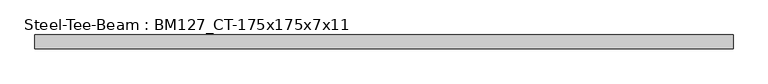
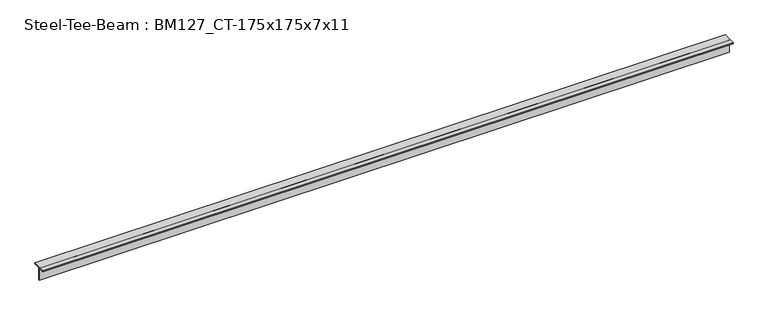
"""IFC4 building model written with IfcOpenShell, lengths in millimetres: beam geometry, Steel-Tee-Beam : BM127_CT-175x175x7x11."""

import ifcopenshell
import ifcopenshell.guid

model = None  # the IFC model being written
_history = None  # IfcOwnerHistory: only IFC2X3 demands one
_inside = {}  # id of a spatial element -> (the spatial element, [elements in it])
_under = {}  # id of a project, library or spatial element -> (it, [spatial elements below it])
_declared = {}  # id of a project -> (the project, [libraries it declares])
_typed = {}  # id of a type object -> (the type object, [elements of that type])
_made_of = {}  # id of a material, layer set ... -> (it, [elements and type objects made of it])


def new_model(schema):
    """Start an empty IFC model of exactly this schema.

    Asked for "IFC4X3", IfcOpenShell would pick the latest addendum, in which some entities
    have other attributes; the version numbers below select the first issue.
    IFC2X3 requires an IfcOwnerHistory on every rooted entity: one is made here for all.
    """
    global model, _history
    if schema == "IFC4X3":
        model = ifcopenshell.file(schema_version=(4, 3, 0, 0))
    else:
        model = ifcopenshell.file(schema=schema)
    _inside.clear()
    _under.clear()
    _declared.clear()
    _typed.clear()
    _made_of.clear()
    _history = None
    if model.schema == "IFC2X3":
        org = make("IfcOrganization", Name="unknown")
        user = make(
            "IfcPersonAndOrganization",
            ThePerson=make("IfcPerson", FamilyName="unknown"),
            TheOrganization=org,
        )
        app = make(
            "IfcApplication",
            ApplicationDeveloper=org,
            Version="unknown",
            ApplicationFullName="unknown",
            ApplicationIdentifier="unknown",
        )
        _history = make(
            "IfcOwnerHistory",
            OwningUser=user,
            OwningApplication=app,
            ChangeAction="ADDED",
            CreationDate=0,
        )
    return model


def make(cls, **values):
    """One entity of the class cls with the attributes given. An attribute that is None is left unset."""
    return model.create_entity(
        cls, **{name: value for name, value in values.items() if value is not None}
    )


def rooted(cls, **values):
    """An entity with a GlobalId (a new one), such as an element, a storey or a relation."""
    return make(cls, GlobalId=ifcopenshell.guid.new(), OwnerHistory=_history, **values)


def si_unit(unit_type, name, prefix=None):
    """IfcSIUnit, for example si_unit("LENGTHUNIT", "METRE", prefix="MILLI")."""
    return make("IfcSIUnit", UnitType=unit_type, Prefix=prefix, Name=name)


def assignment(units):
    """IfcUnitAssignment: the units of a project."""
    return None if units is None else make("IfcUnitAssignment", Units=units)


def point(xyz):
    """IfcCartesianPoint."""
    return None if xyz is None else make("IfcCartesianPoint", Coordinates=xyz)


def direction(xyz):
    """IfcDirection."""
    return None if xyz is None else make("IfcDirection", DirectionRatios=xyz)


def frame(location, z_axis=None, x_axis=None):
    """IfcAxis2Placement3D, a coordinate frame: its origin and axes. An axis left out is left unset."""
    return make(
        "IfcAxis2Placement3D",
        Location=point(location),
        Axis=direction(z_axis),
        RefDirection=direction(x_axis),
    )


def frame_2d(location, x_axis=None):
    """IfcAxis2Placement2D, a coordinate frame in the plane: its origin and x axis."""
    return make(
        "IfcAxis2Placement2D", Location=point(location), RefDirection=direction(x_axis)
    )


def origin():
    """The frame at (0, 0, 0) with its axes left unset."""
    return frame((0.0, 0.0, 0.0))


def place(relative_to, where):
    """IfcLocalPlacement: puts the frame where relative to a parent placement (None: the world)."""
    return make(
        "IfcLocalPlacement", PlacementRelTo=relative_to, RelativePlacement=where
    )


def context(
    kind, dimensions, precision=None, world=None, true_north=None, identifier=None
):
    """IfcGeometricRepresentationContext, for example the 3D "Model" context."""
    return make(
        "IfcGeometricRepresentationContext",
        ContextIdentifier=identifier,
        ContextType=kind,
        CoordinateSpaceDimension=dimensions,
        Precision=precision,
        WorldCoordinateSystem=world,
        TrueNorth=true_north,
    )


def project(units=None, contexts=None):
    """IfcProject with its units and contexts."""
    return rooted(
        "IfcProject",
        Name="project",
        RepresentationContexts=contexts,
        UnitsInContext=assignment(units),
    )


def spatial(cls, under=None, at=None, **own):
    """A site, building, storey or space (cls), placed at a placement, below another one or the project."""
    s = rooted(cls, ObjectPlacement=at, **own)
    if under is not None:
        _under.setdefault(under.id(), (under, []))[1].append(s)
    return s


def polyline(points):
    """IfcPolyline through the points."""
    return make("IfcPolyline", Points=[point(p) for p in points])


def circle_curve(where, radius):
    """IfcCircle in the frame where."""
    return make("IfcCircle", Position=where, Radius=radius)


def trimmed(basis, trim1, trim2, sense, master):
    """IfcTrimmedCurve: the piece of a basis curve between two trims."""
    return make(
        "IfcTrimmedCurve",
        BasisCurve=basis,
        Trim1=trim1,
        Trim2=trim2,
        SenseAgreement=sense,
        MasterRepresentation=master,
    )


def segment(curve, same_sense, transition):
    """IfcCompositeCurveSegment."""
    return make(
        "IfcCompositeCurveSegment",
        Transition=transition,
        SameSense=same_sense,
        ParentCurve=curve,
    )


def composite_curve(segments, self_intersect=None):
    """IfcCompositeCurve: segments joined end to end."""
    return make("IfcCompositeCurve", Segments=segments, SelfIntersect=self_intersect)


def outline(outer, holes=None, kind="AREA"):
    """IfcArbitraryClosedProfileDef: a profile drawn as a closed curve; with holes, ...WithVoids."""
    if holes is None:
        return make("IfcArbitraryClosedProfileDef", ProfileType=kind, OuterCurve=outer)
    return make(
        "IfcArbitraryProfileDefWithVoids",
        ProfileType=kind,
        OuterCurve=outer,
        InnerCurves=holes,
    )


def extrude(swept, where, along, depth):
    """IfcExtrudedAreaSolid: the profile swept, set in the frame where, extruded along a direction by depth."""
    return make(
        "IfcExtrudedAreaSolid",
        SweptArea=swept,
        Position=where,
        ExtrudedDirection=direction(along),
        Depth=depth,
    )


def shape(context_of_items, identifier, shape_type, items):
    """IfcShapeRepresentation: the items that make up one representation, for example the "Body"."""
    return make(
        "IfcShapeRepresentation",
        ContextOfItems=context_of_items,
        RepresentationIdentifier=identifier,
        RepresentationType=shape_type,
        Items=items,
    )


def source(mapping_origin, context_of_items, identifier, shape_type, items):
    """IfcRepresentationMap: a shape defined once, which mapped items show again and again."""
    return make(
        "IfcRepresentationMap",
        MappingOrigin=mapping_origin,
        MappedRepresentation=shape(context_of_items, identifier, shape_type, items),
    )


def transform(
    local_origin,
    x_axis=None,
    y_axis=None,
    z_axis=None,
    scale=None,
    scale2=None,
    scale3=None,
    uniform=True,
):
    """IfcCartesianTransformationOperator3D, or its non-uniform kind. x_axis, y_axis, z_axis: its Axis1, 2, 3."""
    if uniform:
        return make(
            "IfcCartesianTransformationOperator3D",
            Axis1=direction(x_axis),
            Axis2=direction(y_axis),
            LocalOrigin=point(local_origin),
            Scale=scale,
            Axis3=direction(z_axis),
        )
    return make(
        "IfcCartesianTransformationOperator3DnonUniform",
        Axis1=direction(x_axis),
        Axis2=direction(y_axis),
        LocalOrigin=point(local_origin),
        Scale=scale,
        Axis3=direction(z_axis),
        Scale2=scale2,
        Scale3=scale3,
    )


def mapped(mapping_source, mapping_target):
    """IfcMappedItem: shows the shape of a source again, moved by a transform."""
    return make(
        "IfcMappedItem", MappingSource=mapping_source, MappingTarget=mapping_target
    )


def made_of(thing, what):
    """Note that an element or type object is made of a material, layer set ...; save() writes the relation."""
    if what is not None:
        _made_of.setdefault(what.id(), (what, []))[1].append(thing)
    return thing


def element(
    cls,
    number,
    at=None,
    inside=None,
    cuts=None,
    type_object=None,
    material=None,
    context=None,
    identifier="Body",
    shape_type=None,
    held_by="IfcProductDefinitionShape",
    body=None,
    shapes=None,
    **own,
):
    """One element of the class cls, such as IfcWall. Its Tag is "e" and its number.

    at: its placement. inside: the storey or other place that contains it. cuts: it is an
    opening in that element (IfcRelVoidsElement). A single representation is given by context,
    identifier, shape_type and body (its items); several are given by shapes. held_by: the class
    of the entity that holds the representations. save() writes the other relations.
    """
    e = rooted(cls, Tag="e%d" % number, ObjectPlacement=at, **own)
    if body is not None:
        shapes = [shape(context, identifier, shape_type, body)]
    if shapes is not None:
        e.Representation = make(held_by, Representations=shapes)
    if inside is not None:
        _inside.setdefault(inside.id(), (inside, []))[1].append(e)
    if cuts is not None:
        rooted(
            "IfcRelVoidsElement", RelatingBuildingElement=cuts, RelatedOpeningElement=e
        )
    if type_object is not None:
        _typed.setdefault(type_object.id(), (type_object, []))[1].append(e)
    return made_of(e, material)


def aggregate(whole, parts):
    """IfcRelAggregates: a whole, such as a stair, and the parts it consists of."""
    return rooted("IfcRelAggregates", RelatingObject=whole, RelatedObjects=parts)


def save(model, path):
    """Write the relations noted so far, then the file.

    IfcRelAggregates (storeys below a building ...), IfcRelContainedInSpatialStructure (elements
    in a storey), IfcRelDefinesByType, IfcRelAssociatesMaterial and IfcRelDeclares: one each for
    every whole, place, type object, material and project.
    """
    for whole, parts in _under.values():
        aggregate(whole, parts)
    for where, things in _inside.values():
        rooted(
            "IfcRelContainedInSpatialStructure",
            RelatedElements=things,
            RelatingStructure=where,
        )
    for kind, things in _typed.values():
        rooted("IfcRelDefinesByType", RelatedObjects=things, RelatingType=kind)
    for what, things in _made_of.values():
        rooted("IfcRelAssociatesMaterial", RelatedObjects=things, RelatingMaterial=what)
    for by, libraries in _declared.values():
        rooted("IfcRelDeclares", RelatingContext=by, RelatedDefinitions=libraries)
    model.write(path)


def steel_tee_beam_bm127_ct_175x175x7x11_fc6d57d6(model_context):
    return source(origin(), model_context, "Body", "SweptSolid", [
        extrude(outline(composite_curve([segment(polyline([(-87.5, 87.5), (87.5, 87.5), (87.5, 76.5), (17.5, 76.5)]), True, "CONTINUOUS"), segment(trimmed(circle_curve(frame_2d((17.5, 62.5)), 14.0), [point((17.5, 76.5))], [point((3.5, 62.5))], True, "CARTESIAN"), True, "CONTINUOUS"), segment(polyline([(3.5, 62.5), (3.5, -87.5), (-3.5, -87.5), (-3.5, 62.5)]), True, "CONTINUOUS"), segment(trimmed(circle_curve(frame_2d((-17.5, 62.5)), 14.0), [point((-3.5, 62.5))], [point((-17.5, 76.5))], True, "CARTESIAN"), True, "CONTINUOUS"), segment(polyline([(-17.5, 76.5), (-87.5, 76.5), (-87.5, 87.5)]), True, "CONTINUOUS")], self_intersect=False)), frame((-4298.1792655, 0.0, 0.0), z_axis=(1.0, 0.0, 0.0), x_axis=(0.0, 1.0, 0.0)), (0.0, 0.0, 1.0), 8725.555017),
    ])


if __name__ == "__main__":
    model = new_model("IFC4")
    model_context = context("Model", 3, world=origin())
    ifc_project = project(units=[si_unit("LENGTHUNIT", "METRE", prefix="MILLI")], contexts=[model_context])
    site = spatial("IfcSite", under=ifc_project)
    building = spatial("IfcBuilding", under=site)
    placement = place(None, origin())
    steel_tee_beam_bm127_ct_175x175x7x11_shape = steel_tee_beam_bm127_ct_175x175x7x11_fc6d57d6(model_context)
    element("IfcBeam", 1, ObjectType="Steel-Tee-Beam : BM127_CT-175x175x7x11", at=placement, inside=building, context=model_context, shape_type="MappedRepresentation", body=[
        mapped(steel_tee_beam_bm127_ct_175x175x7x11_shape, transform((0.0, 0.0, 0.0), x_axis=(1.0, 0.0, 0.0), y_axis=(0.0, 1.0, 0.0), z_axis=(0.0, 0.0, 1.0))),
    ])
    save(model, "model.ifc")

# Revit data of these elements
# Type "Steel-Tee-Beam : BM127_CT-175x175x7x11"
#   Surface Area = 0.00 m²/m
#   Section Area = 31.57 cm²
#   Mass per Unit Length = 24.80 kg/m
#   Length [instance default] = 1524 mm
#   bf = 175 mm
#   d = 175 mm
#   k = 25 mm
#   kr = 14 mm
#   tf = 11 mm
#   tw = 7 mm
#   hec_material4 [instance default] = none
#   hec_material3 [instance default] = none
#   hec_material2 [instance default] = none
#   hec_material1 [instance default] = none
#   Structural Material [instance default] = Steel, 45-345
#   Assembly Code = ""
# Element 1 (IfcBeam, "Steel-Tee-Beam : BM127_CT-175x175x7x11")
#   hec_material3 = F01AC000-00002_Building/Shelter Fire Proofing Work_Intumescent Coating Type_1 hr. rating (UL 1709))
#   hec_material2 = S01AA010-00002_Main Steel Structure Fabrication Work_Shelter/Building_Steel Painting/Coating_for Fireproofed Steel Surface, Surface Preparation & Primer Coat
#   hec_material1 = S03AA029-00001_Main Steel Structure Erection Work_Shelter/Building_Light Steel
#   Structural Material = S01AA003-00001_Main Steel Structure Fabrication Work_Shelter/Building_Light Steel - Standard
#   Materials on its faces: "S01AA003-00001_Main Steel Structure Fabrication Work_Shelter/Building_Light Steel - Standard"
# Materials
#   "Steel, 45-345": class "Metal", colour RGB 189 187 185, transparency 0, Description = "Steel 345 MPa", Cost = 0
#   "S01AA003-00001_Main Steel Structure Fabrication Work_Shelter/Building_Light Steel - Standard": class "Metal", colour RGB 120 120 120, transparency 0, Comments = "(30KG/M>Weight)", Description = "Structural steel 50ksi", W00) Work Master Code = "S01AA003-00001", W01) Work Master_Lv1 = "Main Steel Structure Fabrication Work", W02) Work Master_Lv2 = "Shelter/Building", W03) Work Master_Spec.1 = "Light Steel - Standard (30KG/M>Weight)", Cost = 0
#   "F01AC000-00002_Building/Shelter Fire Proofing Work_Intumescent Coating Type_1 hr. rating (UL 1709))": class "Metal", colour RGB 255 128 128, transparency 0, Description = "Paint finished steel", W00) Work Master Code = "F01AC000-00002", W01) Work Master_Lv1 = "Building/Shelter Fire Proofing Work", W02) Work Master_Lv2 = "Intumescent Coating Type", W03) Work Master_Spec.1 = "1 hr. rating (UL 1709)", Cost = 0
#   "S01AA010-00002_Main Steel Structure Fabrication Work_Shelter/Building_Steel Painting/Coating_for Fireproofed Steel Surface, Surface Preparation & Primer Coat": class "Metal", colour RGB 120 120 120, transparency 0, Description = "Paint finished steel", W00) Work Master Code = "SS01AA010-00002", W01) Work Master_Lv1 = "Main Steel Structure Fabrication Work", W02) Work Master_Lv2 = "Shelter/Building", W03) Work Master_Spec.1 = "Steel Painting/Coating", W04) Work Master_Spec.2 = "for Fireproofed Steel Surface, Surface Preparation & Primer Coat", Cost = 0
#   "S03AA029-00001_Main Steel Structure Erection Work_Shelter/Building_Light Steel": class "Metal", colour RGB 120 120 120, transparency 0, Comments = "(30KG/M>Weight)", Description = "Structural steel 50ksi", W00) Work Master Code = "S03AA029-00001", W01) Work Master_Lv1 = "Main Steel Structure Erection Work", W02) Work Master_Lv2 = "Shelter/Building", W03) Work Master_Spec.1 = "Light Steel (30KG/M>Weight)", Cost = 0
